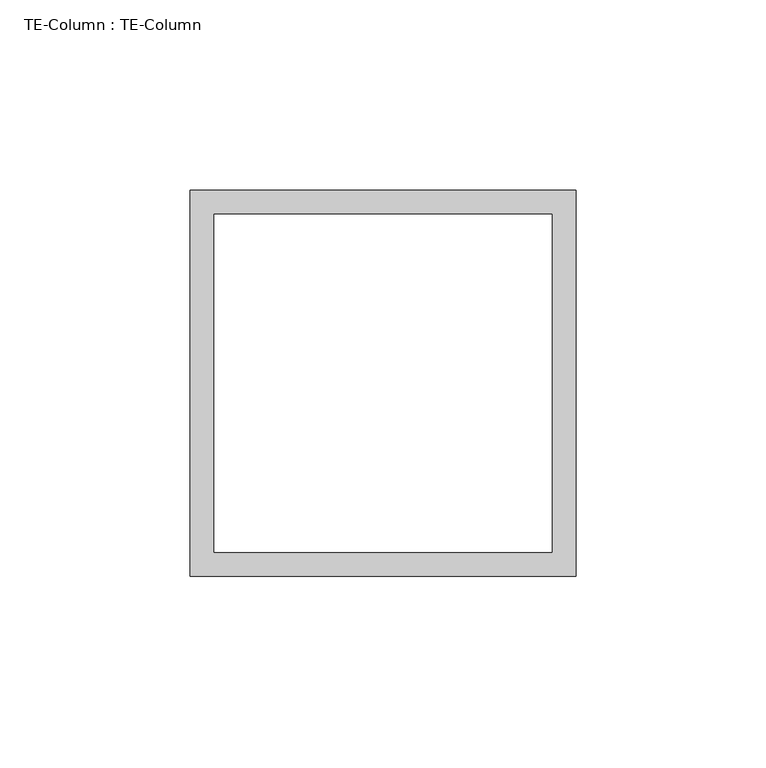
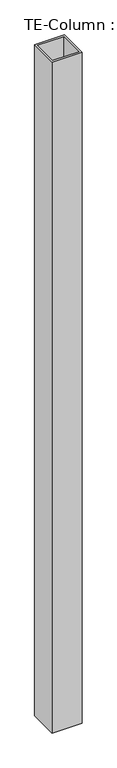
"""IFC4 building model written with IfcOpenShell, lengths in millimetres: proxy geometry, TE-Column : TE-Column."""

from ifc_helpers import new_model, si_unit, frame, origin, place, context, project, spatial, polyline, outline, extrude, source, transform, mapped, element, save


def te_column_te_column_7b45b3bc(model_context):
    return source(origin(), model_context, "Body", "SweptSolid", [
        extrude(outline(polyline([(587467.4934739, -531667.7913841), (587467.4934739, -531769.3913841), (587365.8934739, -531769.3913841), (587365.8934739, -531667.7913841), (587467.4934739, -531667.7913841)]), holes=[polyline([(587372.2434739, -531674.1413841), (587372.2434739, -531763.0413841), (587461.1434739, -531763.0413841), (587461.1434739, -531674.1413841), (587372.2434739, -531674.1413841)])]), frame((0.0, 0.0, 28.575), z_axis=(0.0, 0.0, 1.0), x_axis=(1.0, 0.0, 0.0)), (0.0, 0.0, 1.0), 2406.65),
    ])


if __name__ == "__main__":
    model = new_model("IFC4")
    model_context = context("Model", 3, world=origin())
    ifc_project = project(units=[si_unit("LENGTHUNIT", "METRE", prefix="MILLI")], contexts=[model_context])
    site = spatial("IfcSite", under=ifc_project)
    building = spatial("IfcBuilding", under=site)
    placement = place(None, origin())
    te_column_te_column_shape = te_column_te_column_7b45b3bc(model_context)
    element("IfcBuildingElementProxy", 1, Name="TE-Column : TE-Column", ObjectType="TE-Column : TE-Column", at=placement, inside=building, context=model_context, shape_type="MappedRepresentation", body=[
        mapped(te_column_te_column_shape, transform((0.0, 0.0, 0.0), x_axis=(1.0, 0.0, 0.0), y_axis=(0.0, 1.0, 0.0), z_axis=(0.0, 0.0, 1.0))),
    ])
    save(model, "model.ifc")

# Revit data of these elements
# Element 1 (IfcBuildingElementProxy, "TE-Column : TE-Column")
#   Materials on its faces: "4\"X4\" GALV. HSS TUBING"
# Materials
#   "4\"X4\" GALV. HSS TUBING": class "Generic", colour RGB 211 211 207, transparency 0, Cost = 0
